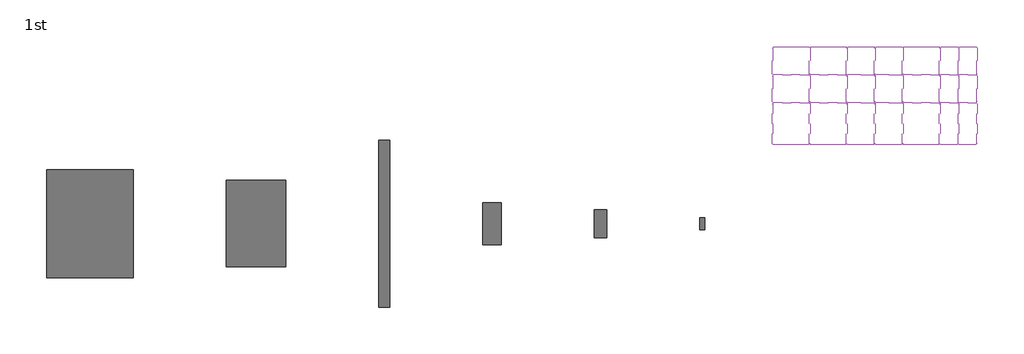
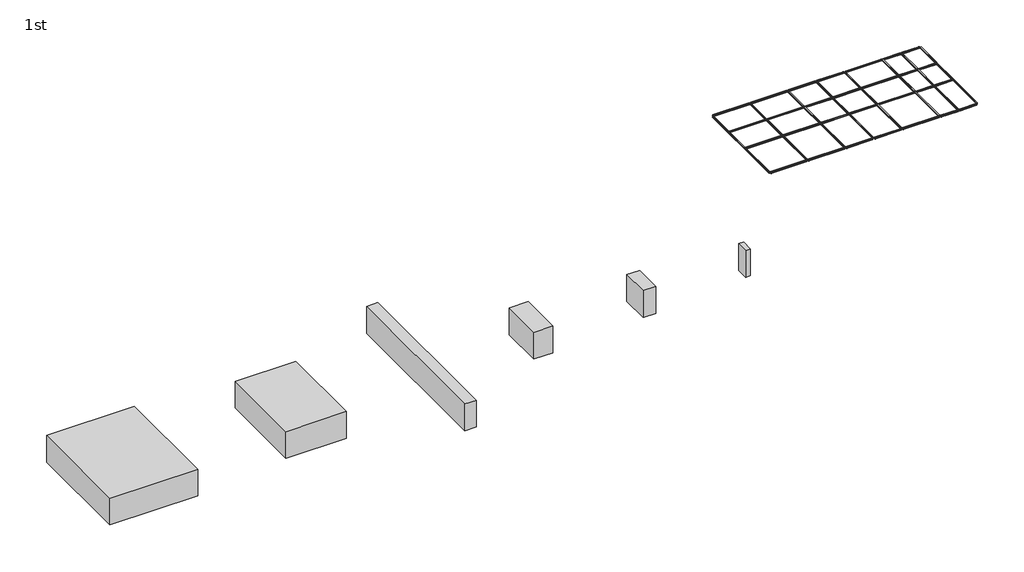
# One storey: 52 beams, 6 proxies.
"""IFC4 building model written with IfcOpenShell, lengths in millimetres."""

import ifcopenshell
import ifcopenshell.guid

model = None  # the IFC model being written
_history = None  # IfcOwnerHistory: only IFC2X3 demands one
_inside = {}  # id of a spatial element -> (the spatial element, [elements in it])
_under = {}  # id of a project, library or spatial element -> (it, [spatial elements below it])
_declared = {}  # id of a project -> (the project, [libraries it declares])
_typed = {}  # id of a type object -> (the type object, [elements of that type])
_made_of = {}  # id of a material, layer set ... -> (it, [elements and type objects made of it])


def new_model(schema):
    """Start an empty IFC model of exactly this schema.

    Asked for "IFC4X3", IfcOpenShell would pick the latest addendum, in which some entities
    have other attributes; the version numbers below select the first issue.
    IFC2X3 requires an IfcOwnerHistory on every rooted entity: one is made here for all.
    """
    global model, _history
    if schema == "IFC4X3":
        model = ifcopenshell.file(schema_version=(4, 3, 0, 0))
    else:
        model = ifcopenshell.file(schema=schema)
    _inside.clear()
    _under.clear()
    _declared.clear()
    _typed.clear()
    _made_of.clear()
    _history = None
    if model.schema == "IFC2X3":
        org = make("IfcOrganization", Name="unknown")
        user = make(
            "IfcPersonAndOrganization",
            ThePerson=make("IfcPerson", FamilyName="unknown"),
            TheOrganization=org,
        )
        app = make(
            "IfcApplication",
            ApplicationDeveloper=org,
            Version="unknown",
            ApplicationFullName="unknown",
            ApplicationIdentifier="unknown",
        )
        _history = make(
            "IfcOwnerHistory",
            OwningUser=user,
            OwningApplication=app,
            ChangeAction="ADDED",
            CreationDate=0,
        )
    return model


def make(cls, **values):
    """One entity of the class cls with the attributes given. An attribute that is None is left unset."""
    return model.create_entity(
        cls, **{name: value for name, value in values.items() if value is not None}
    )


def rooted(cls, **values):
    """An entity with a GlobalId (a new one), such as an element, a storey or a relation."""
    return make(cls, GlobalId=ifcopenshell.guid.new(), OwnerHistory=_history, **values)


def si_unit(unit_type, name, prefix=None):
    """IfcSIUnit, for example si_unit("LENGTHUNIT", "METRE", prefix="MILLI")."""
    return make("IfcSIUnit", UnitType=unit_type, Prefix=prefix, Name=name)


def assignment(units):
    """IfcUnitAssignment: the units of a project."""
    return None if units is None else make("IfcUnitAssignment", Units=units)


def point(xyz):
    """IfcCartesianPoint."""
    return None if xyz is None else make("IfcCartesianPoint", Coordinates=xyz)


def direction(xyz):
    """IfcDirection."""
    return None if xyz is None else make("IfcDirection", DirectionRatios=xyz)


def frame(location, z_axis=None, x_axis=None):
    """IfcAxis2Placement3D, a coordinate frame: its origin and axes. An axis left out is left unset."""
    return make(
        "IfcAxis2Placement3D",
        Location=point(location),
        Axis=direction(z_axis),
        RefDirection=direction(x_axis),
    )


def frame_2d(location, x_axis=None):
    """IfcAxis2Placement2D, a coordinate frame in the plane: its origin and x axis."""
    return make(
        "IfcAxis2Placement2D", Location=point(location), RefDirection=direction(x_axis)
    )


def origin():
    """The frame at (0, 0, 0) with its axes left unset."""
    return frame((0.0, 0.0, 0.0))


def origin_with_axes():
    """The frame at (0, 0, 0) with the z axis (0, 0, 1) and the x axis (1, 0, 0) written out."""
    return frame((0.0, 0.0, 0.0), z_axis=(0.0, 0.0, 1.0), x_axis=(1.0, 0.0, 0.0))


def place(relative_to, where):
    """IfcLocalPlacement: puts the frame where relative to a parent placement (None: the world)."""
    return make(
        "IfcLocalPlacement", PlacementRelTo=relative_to, RelativePlacement=where
    )


def context(
    kind, dimensions, precision=None, world=None, true_north=None, identifier=None
):
    """IfcGeometricRepresentationContext, for example the 3D "Model" context."""
    return make(
        "IfcGeometricRepresentationContext",
        ContextIdentifier=identifier,
        ContextType=kind,
        CoordinateSpaceDimension=dimensions,
        Precision=precision,
        WorldCoordinateSystem=world,
        TrueNorth=true_north,
    )


def project(units=None, contexts=None):
    """IfcProject with its units and contexts."""
    return rooted(
        "IfcProject",
        Name="project",
        RepresentationContexts=contexts,
        UnitsInContext=assignment(units),
    )


def spatial(cls, under=None, at=None, **own):
    """A site, building, storey or space (cls), placed at a placement, below another one or the project."""
    s = rooted(cls, ObjectPlacement=at, **own)
    if under is not None:
        _under.setdefault(under.id(), (under, []))[1].append(s)
    return s


def polyline(points):
    """IfcPolyline through the points."""
    return make("IfcPolyline", Points=[point(p) for p in points])


def circle_curve(where, radius):
    """IfcCircle in the frame where."""
    return make("IfcCircle", Position=where, Radius=radius)


def trimmed(basis, trim1, trim2, sense, master):
    """IfcTrimmedCurve: the piece of a basis curve between two trims."""
    return make(
        "IfcTrimmedCurve",
        BasisCurve=basis,
        Trim1=trim1,
        Trim2=trim2,
        SenseAgreement=sense,
        MasterRepresentation=master,
    )


def segment(curve, same_sense, transition):
    """IfcCompositeCurveSegment."""
    return make(
        "IfcCompositeCurveSegment",
        Transition=transition,
        SameSense=same_sense,
        ParentCurve=curve,
    )


def composite_curve(segments, self_intersect=None):
    """IfcCompositeCurve: segments joined end to end."""
    return make("IfcCompositeCurve", Segments=segments, SelfIntersect=self_intersect)


def outline(outer, holes=None, kind="AREA"):
    """IfcArbitraryClosedProfileDef: a profile drawn as a closed curve; with holes, ...WithVoids."""
    if holes is None:
        return make("IfcArbitraryClosedProfileDef", ProfileType=kind, OuterCurve=outer)
    return make(
        "IfcArbitraryProfileDefWithVoids",
        ProfileType=kind,
        OuterCurve=outer,
        InnerCurves=holes,
    )


def extrude(swept, where, along, depth):
    """IfcExtrudedAreaSolid: the profile swept, set in the frame where, extruded along a direction by depth."""
    return make(
        "IfcExtrudedAreaSolid",
        SweptArea=swept,
        Position=where,
        ExtrudedDirection=direction(along),
        Depth=depth,
    )


def shape(context_of_items, identifier, shape_type, items):
    """IfcShapeRepresentation: the items that make up one representation, for example the "Body"."""
    return make(
        "IfcShapeRepresentation",
        ContextOfItems=context_of_items,
        RepresentationIdentifier=identifier,
        RepresentationType=shape_type,
        Items=items,
    )


def source(mapping_origin, context_of_items, identifier, shape_type, items):
    """IfcRepresentationMap: a shape defined once, which mapped items show again and again."""
    return make(
        "IfcRepresentationMap",
        MappingOrigin=mapping_origin,
        MappedRepresentation=shape(context_of_items, identifier, shape_type, items),
    )


def transform(
    local_origin,
    x_axis=None,
    y_axis=None,
    z_axis=None,
    scale=None,
    scale2=None,
    scale3=None,
    uniform=True,
):
    """IfcCartesianTransformationOperator3D, or its non-uniform kind. x_axis, y_axis, z_axis: its Axis1, 2, 3."""
    if uniform:
        return make(
            "IfcCartesianTransformationOperator3D",
            Axis1=direction(x_axis),
            Axis2=direction(y_axis),
            LocalOrigin=point(local_origin),
            Scale=scale,
            Axis3=direction(z_axis),
        )
    return make(
        "IfcCartesianTransformationOperator3DnonUniform",
        Axis1=direction(x_axis),
        Axis2=direction(y_axis),
        LocalOrigin=point(local_origin),
        Scale=scale,
        Axis3=direction(z_axis),
        Scale2=scale2,
        Scale3=scale3,
    )


def mapped(mapping_source, mapping_target):
    """IfcMappedItem: shows the shape of a source again, moved by a transform."""
    return make(
        "IfcMappedItem", MappingSource=mapping_source, MappingTarget=mapping_target
    )


def made_of(thing, what):
    """Note that an element or type object is made of a material, layer set ...; save() writes the relation."""
    if what is not None:
        _made_of.setdefault(what.id(), (what, []))[1].append(thing)
    return thing


def element(
    cls,
    number,
    at=None,
    inside=None,
    cuts=None,
    type_object=None,
    material=None,
    context=None,
    identifier="Body",
    shape_type=None,
    held_by="IfcProductDefinitionShape",
    body=None,
    shapes=None,
    **own,
):
    """One element of the class cls, such as IfcWall. Its Tag is "e" and its number.

    at: its placement. inside: the storey or other place that contains it. cuts: it is an
    opening in that element (IfcRelVoidsElement). A single representation is given by context,
    identifier, shape_type and body (its items); several are given by shapes. held_by: the class
    of the entity that holds the representations. save() writes the other relations.
    """
    e = rooted(cls, Tag="e%d" % number, ObjectPlacement=at, **own)
    if body is not None:
        shapes = [shape(context, identifier, shape_type, body)]
    if shapes is not None:
        e.Representation = make(held_by, Representations=shapes)
    if inside is not None:
        _inside.setdefault(inside.id(), (inside, []))[1].append(e)
    if cuts is not None:
        rooted(
            "IfcRelVoidsElement", RelatingBuildingElement=cuts, RelatedOpeningElement=e
        )
    if type_object is not None:
        _typed.setdefault(type_object.id(), (type_object, []))[1].append(e)
    return made_of(e, material)


def aggregate(whole, parts):
    """IfcRelAggregates: a whole, such as a stair, and the parts it consists of."""
    return rooted("IfcRelAggregates", RelatingObject=whole, RelatedObjects=parts)


def save(model, path):
    """Write the relations noted so far, then the file.

    IfcRelAggregates (storeys below a building ...), IfcRelContainedInSpatialStructure (elements
    in a storey), IfcRelDefinesByType, IfcRelAssociatesMaterial and IfcRelDeclares: one each for
    every whole, place, type object, material and project.
    """
    for whole, parts in _under.values():
        aggregate(whole, parts)
    for where, things in _inside.values():
        rooted(
            "IfcRelContainedInSpatialStructure",
            RelatedElements=things,
            RelatingStructure=where,
        )
    for kind, things in _typed.values():
        rooted("IfcRelDefinesByType", RelatedObjects=things, RelatingType=kind)
    for what, things in _made_of.values():
        rooted("IfcRelAssociatesMaterial", RelatedObjects=things, RelatingMaterial=what)
    for by, libraries in _declared.values():
        rooted("IfcRelDeclares", RelatingContext=by, RelatedDefinitions=libraries)
    model.write(path)


def ub_universal_beams_ub305x165x40_6dcc7521(model_context):
    return source(origin(), model_context, "Body", "SweptSolid", [
        extrude(outline(composite_curve([segment(polyline([(82.5, -141.5), (82.5, -151.7), (-82.5, -151.7), (-82.5, -141.5), (-11.9, -141.5)]), True, "CONTINUOUS"), segment(trimmed(circle_curve(frame_2d((-11.9, -132.6)), 8.9), [point((-11.9, -141.5))], [point((-3.0, -132.6))], True, "CARTESIAN"), True, "CONTINUOUS"), segment(polyline([(-3.0, -132.6), (-3.0, 132.6)]), True, "CONTINUOUS"), segment(trimmed(circle_curve(frame_2d((-11.9, 132.6)), 8.9), [point((-3.0, 132.6))], [point((-11.9, 141.5))], True, "CARTESIAN"), True, "CONTINUOUS"), segment(polyline([(-11.9, 141.5), (-82.5, 141.5), (-82.5, 151.7), (82.5, 151.7), (82.5, 141.5), (11.9, 141.5)]), True, "CONTINUOUS"), segment(trimmed(circle_curve(frame_2d((11.9, 132.6)), 8.9), [point((11.9, 141.5))], [point((3.0, 132.6))], True, "CARTESIAN"), True, "CONTINUOUS"), segment(polyline([(3.0, 132.6), (3.0, -132.6)]), True, "CONTINUOUS"), segment(trimmed(circle_curve(frame_2d((11.9, -132.6)), 8.9), [point((3.0, -132.6))], [point((11.9, -141.5))], True, "CARTESIAN"), True, "CONTINUOUS"), segment(polyline([(11.9, -141.5), (82.5, -141.5)]), True, "CONTINUOUS")], self_intersect=False)), frame((-4333.3, 0.0, 0.0), z_axis=(1.0, 0.0, 0.0), x_axis=(0.0, 1.0, 0.0)), (0.0, 0.0, 1.0), 8666.6),
    ])


def ub_universal_beams_ub305x165x40_7f5f946b(model_context):
    return source(origin(), model_context, "Body", "SweptSolid", [
        extrude(outline(composite_curve([segment(polyline([(82.5, -141.5), (82.5, -151.7), (-82.5, -151.7), (-82.5, -141.5), (-11.9, -141.5)]), True, "CONTINUOUS"), segment(trimmed(circle_curve(frame_2d((-11.9, -132.6)), 8.9), [point((-11.9, -141.5))], [point((-3.0, -132.6))], True, "CARTESIAN"), True, "CONTINUOUS"), segment(polyline([(-3.0, -132.6), (-3.0, 132.6)]), True, "CONTINUOUS"), segment(trimmed(circle_curve(frame_2d((-11.9, 132.6)), 8.9), [point((-3.0, 132.6))], [point((-11.9, 141.5))], True, "CARTESIAN"), True, "CONTINUOUS"), segment(polyline([(-11.9, 141.5), (-82.5, 141.5), (-82.5, 151.7), (82.5, 151.7), (82.5, 141.5), (11.9, 141.5)]), True, "CONTINUOUS"), segment(trimmed(circle_curve(frame_2d((11.9, 132.6)), 8.9), [point((11.9, 141.5))], [point((3.0, 132.6))], True, "CARTESIAN"), True, "CONTINUOUS"), segment(polyline([(3.0, 132.6), (3.0, -132.6)]), True, "CONTINUOUS"), segment(trimmed(circle_curve(frame_2d((11.9, -132.6)), 8.9), [point((3.0, -132.6))], [point((11.9, -141.5))], True, "CARTESIAN"), True, "CONTINUOUS"), segment(polyline([(11.9, -141.5), (82.5, -141.5)]), True, "CONTINUOUS")], self_intersect=False)), frame((-2833.3, 0.0, 0.0), z_axis=(1.0, 0.0, 0.0), x_axis=(0.0, 1.0, 0.0)), (0.0, 0.0, 1.0), 5666.6),
    ])


def ub_universal_beams_ub305x165x40_37dc1813(model_context):
    return source(origin(), model_context, "Body", "SweptSolid", [
        extrude(outline(composite_curve([segment(polyline([(82.5, -141.5), (82.5, -151.7), (-82.5, -151.7), (-82.5, -141.5), (-11.9, -141.5)]), True, "CONTINUOUS"), segment(trimmed(circle_curve(frame_2d((-11.9, -132.6)), 8.9), [point((-11.9, -141.5))], [point((-3.0, -132.6))], True, "CARTESIAN"), True, "CONTINUOUS"), segment(polyline([(-3.0, -132.6), (-3.0, 132.6)]), True, "CONTINUOUS"), segment(trimmed(circle_curve(frame_2d((-11.9, 132.6)), 8.9), [point((-3.0, 132.6))], [point((-11.9, 141.5))], True, "CARTESIAN"), True, "CONTINUOUS"), segment(polyline([(-11.9, 141.5), (-82.5, 141.5), (-82.5, 151.7), (82.5, 151.7), (82.5, 141.5), (11.9, 141.5)]), True, "CONTINUOUS"), segment(trimmed(circle_curve(frame_2d((11.9, 132.6)), 8.9), [point((11.9, 141.5))], [point((3.0, 132.6))], True, "CARTESIAN"), True, "CONTINUOUS"), segment(polyline([(3.0, 132.6), (3.0, -132.6)]), True, "CONTINUOUS"), segment(trimmed(circle_curve(frame_2d((11.9, -132.6)), 8.9), [point((3.0, -132.6))], [point((11.9, -141.5))], True, "CARTESIAN"), True, "CONTINUOUS"), segment(polyline([(11.9, -141.5), (82.5, -141.5)]), True, "CONTINUOUS")], self_intersect=False)), frame((-3834.6, 0.0, 0.0), z_axis=(1.0, 0.0, 0.0), x_axis=(0.0, 1.0, 0.0)), (0.0, 0.0, 1.0), 7669.2),
    ])


def ub_universal_beams_ub305x165x40_4fbda082(model_context):
    return source(origin(), model_context, "Body", "SweptSolid", [
        extrude(outline(composite_curve([segment(polyline([(82.5, -141.5), (82.5, -151.7), (-82.5, -151.7), (-82.5, -141.5), (-11.9, -141.5)]), True, "CONTINUOUS"), segment(trimmed(circle_curve(frame_2d((-11.9, -132.6)), 8.9), [point((-11.9, -141.5))], [point((-3.0, -132.6))], True, "CARTESIAN"), True, "CONTINUOUS"), segment(polyline([(-3.0, -132.6), (-3.0, 132.6)]), True, "CONTINUOUS"), segment(trimmed(circle_curve(frame_2d((-11.9, 132.6)), 8.9), [point((-3.0, 132.6))], [point((-11.9, 141.5))], True, "CARTESIAN"), True, "CONTINUOUS"), segment(polyline([(-11.9, 141.5), (-82.5, 141.5), (-82.5, 151.7), (82.5, 151.7), (82.5, 141.5), (11.9, 141.5)]), True, "CONTINUOUS"), segment(trimmed(circle_curve(frame_2d((11.9, 132.6)), 8.9), [point((11.9, 141.5))], [point((3.0, 132.6))], True, "CARTESIAN"), True, "CONTINUOUS"), segment(polyline([(3.0, 132.6), (3.0, -132.6)]), True, "CONTINUOUS"), segment(trimmed(circle_curve(frame_2d((11.9, -132.6)), 8.9), [point((3.0, -132.6))], [point((11.9, -141.5))], True, "CARTESIAN"), True, "CONTINUOUS"), segment(polyline([(11.9, -141.5), (82.5, -141.5)]), True, "CONTINUOUS")], self_intersect=False)), frame((-2834.6, 0.0, 0.0), z_axis=(1.0, 0.0, 0.0), x_axis=(0.0, 1.0, 0.0)), (0.0, 0.0, 1.0), 5669.2),
    ])


def ub_universal_beams_ub305x165x40_037cda9e(model_context):
    return source(origin(), model_context, "Body", "SweptSolid", [
        extrude(outline(composite_curve([segment(polyline([(82.5, -141.5), (82.5, -151.7), (-82.5, -151.7), (-82.5, -141.5), (-11.9, -141.5)]), True, "CONTINUOUS"), segment(trimmed(circle_curve(frame_2d((-11.9, -132.6)), 8.9), [point((-11.9, -141.5))], [point((-3.0, -132.6))], True, "CARTESIAN"), True, "CONTINUOUS"), segment(polyline([(-3.0, -132.6), (-3.0, 132.6)]), True, "CONTINUOUS"), segment(trimmed(circle_curve(frame_2d((-11.9, 132.6)), 8.9), [point((-3.0, 132.6))], [point((-11.9, 141.5))], True, "CARTESIAN"), True, "CONTINUOUS"), segment(polyline([(-11.9, 141.5), (-82.5, 141.5), (-82.5, 151.7), (82.5, 151.7), (82.5, 141.5), (11.9, 141.5)]), True, "CONTINUOUS"), segment(trimmed(circle_curve(frame_2d((11.9, 132.6)), 8.9), [point((11.9, 141.5))], [point((3.0, 132.6))], True, "CARTESIAN"), True, "CONTINUOUS"), segment(polyline([(3.0, 132.6), (3.0, -132.6)]), True, "CONTINUOUS"), segment(trimmed(circle_curve(frame_2d((11.9, -132.6)), 8.9), [point((3.0, -132.6))], [point((11.9, -141.5))], True, "CARTESIAN"), True, "CONTINUOUS"), segment(polyline([(11.9, -141.5), (82.5, -141.5)]), True, "CONTINUOUS")], self_intersect=False)), frame((-1834.6, 0.0, 0.0), z_axis=(1.0, 0.0, 0.0), x_axis=(0.0, 1.0, 0.0)), (0.0, 0.0, 1.0), 3669.2),
    ])


def generic_models_29bcd6f9(model_context):
    return source(origin(), model_context, "Body", "SweptSolid", [
        extrude(outline(polyline([(2000.0, 4500.0), (2000.0, -4500.0), (-2000.0, -4500.0), (-2000.0, 4500.0), (2000.0, 4500.0)])), origin_with_axes(), (0.0, 0.0, 1.0), 6000.0),
    ])


def generic_models_d82b1902(model_context):
    return source(origin(), model_context, "Body", "SweptSolid", [
        extrude(outline(polyline([(9300.0, 11600.0), (9300.0, -11600.0), (-9300.0, -11600.0), (-9300.0, 11600.0), (9300.0, 11600.0)])), origin_with_axes(), (0.0, 0.0, 1.0), 6000.0),
    ])


def generic_models_21711933(model_context):
    return source(origin(), model_context, "Body", "SweptSolid", [
        extrude(outline(polyline([(6400.0, 9300.0), (6400.0, -9300.0), (-6400.0, -9300.0), (-6400.0, 9300.0), (6400.0, 9300.0)])), origin_with_axes(), (0.0, 0.0, 1.0), 6000.0),
    ])


def generic_models_03d31222(model_context):
    return source(origin(), model_context, "Body", "SweptSolid", [
        extrude(outline(polyline([(1200.0, 18000.0), (1200.0, -18000.0), (-1200.0, -18000.0), (-1200.0, 18000.0), (1200.0, 18000.0)])), origin_with_axes(), (0.0, 0.0, 1.0), 6000.0),
    ])


def generic_models_5634f436(model_context):
    return source(origin(), model_context, "Body", "SweptSolid", [
        extrude(outline(polyline([(1350.0, 3000.0), (1350.0, -3000.0), (-1350.0, -3000.0), (-1350.0, 3000.0), (1350.0, 3000.0)])), origin_with_axes(), (0.0, 0.0, 1.0), 6000.0),
    ])


def generic_models_71e2440f(model_context):
    return source(origin(), model_context, "Body", "SweptSolid", [
        extrude(outline(polyline([(500.0, 1250.0), (500.0, -1250.0), (-500.0, -1250.0), (-500.0, 1250.0), (500.0, 1250.0)])), origin_with_axes(), (0.0, 0.0, 1.0), 6000.0),
    ])


model = new_model("IFC4")

# Units and contexts
model_context = context("Model", 3, world=origin())
ifc_project = project(units=[si_unit("LENGTHUNIT", "METRE", prefix="MILLI")], contexts=[model_context])

# Site, building, storey
site = spatial("IfcSite", under=ifc_project)
building = spatial("IfcBuilding", under=site)
storey = spatial("IfcBuildingStorey", under=building, Name="1st", Elevation=7000.0)

# Beams
placement = place(None, origin())
ub_universal_beams_ub305x165x40_shape = ub_universal_beams_ub305x165x40_6dcc7521(model_context)
element("IfcBeam", 1, ObjectType="UB-Universal Beams : UB305x165x40", at=placement, inside=storey, context=model_context, shape_type="MappedRepresentation", body=[
    mapped(ub_universal_beams_ub305x165x40_shape, transform((156114.1020501, 135515.7581198, 13848.3), x_axis=(0.0, 1.0, 0.0), y_axis=(-1.0, 0.0, 0.0), z_axis=(0.0, 0.0, 1.0))),
])
element("IfcBeam", 2, ObjectType="UB-Universal Beams : UB305x165x40", at=placement, inside=storey, context=model_context, shape_type="MappedRepresentation", body=[
    mapped(ub_universal_beams_ub305x165x40_shape, transform((164114.1020501, 135515.7581198, 13848.3), x_axis=(0.0, 1.0, 0.0), y_axis=(-1.0, 0.0, 0.0), z_axis=(0.0, 0.0, 1.0))),
])
element("IfcBeam", 3, ObjectType="UB-Universal Beams : UB305x165x40", at=placement, inside=storey, context=model_context, shape_type="MappedRepresentation", body=[
    mapped(ub_universal_beams_ub305x165x40_shape, transform((172114.1020501, 135515.7581198, 13848.3), x_axis=(0.0, 1.0, 0.0), y_axis=(-1.0, 0.0, 0.0), z_axis=(0.0, 0.0, 1.0))),
])
element("IfcBeam", 4, ObjectType="UB-Universal Beams : UB305x165x40", at=placement, inside=storey, context=model_context, shape_type="MappedRepresentation", body=[
    mapped(ub_universal_beams_ub305x165x40_shape, transform((178114.1020501, 135515.7581198, 13848.3), x_axis=(0.0, 1.0, 0.0), y_axis=(-1.0, 0.0, 0.0), z_axis=(0.0, 0.0, 1.0))),
])
element("IfcBeam", 5, ObjectType="UB-Universal Beams : UB305x165x40", at=placement, inside=storey, context=model_context, shape_type="MappedRepresentation", body=[
    mapped(ub_universal_beams_ub305x165x40_shape, transform((184114.1020501, 135515.7581198, 13848.3), x_axis=(0.0, 1.0, 0.0), y_axis=(-1.0, 0.0, 0.0), z_axis=(0.0, 0.0, 1.0))),
])
element("IfcBeam", 6, ObjectType="UB-Universal Beams : UB305x165x40", at=placement, inside=storey, context=model_context, shape_type="MappedRepresentation", body=[
    mapped(ub_universal_beams_ub305x165x40_shape, transform((192114.1020501, 135515.7581198, 13848.3), x_axis=(0.0, 1.0, 0.0), y_axis=(-1.0, 0.0, 0.0), z_axis=(0.0, 0.0, 1.0))),
])
element("IfcBeam", 7, ObjectType="UB-Universal Beams : UB305x165x40", at=placement, inside=storey, context=model_context, shape_type="MappedRepresentation", body=[
    mapped(ub_universal_beams_ub305x165x40_shape, transform((196114.1020501, 135515.7581198, 13848.3), x_axis=(0.0, 1.0, 0.0), y_axis=(-1.0, 0.0, 0.0), z_axis=(0.0, 0.0, 1.0))),
])
element("IfcBeam", 8, ObjectType="UB-Universal Beams : UB305x165x40", at=placement, inside=storey, context=model_context, shape_type="MappedRepresentation", body=[
    mapped(ub_universal_beams_ub305x165x40_shape, transform((200114.1020501, 135515.7581198, 13848.3), x_axis=(0.0, 1.0, 0.0), y_axis=(-1.0, 0.0, 0.0), z_axis=(0.0, 0.0, 1.0))),
])
ub_universal_beams_ub305x165x40_2_shape = ub_universal_beams_ub305x165x40_7f5f946b(model_context)
element("IfcBeam", 9, ObjectType="UB-Universal Beams : UB305x165x40", at=placement, inside=storey, context=model_context, shape_type="MappedRepresentation", body=[
    mapped(ub_universal_beams_ub305x165x40_2_shape, transform((156114.1020501, 143015.7581198, 13848.3), x_axis=(0.0, 1.0, 0.0), y_axis=(-1.0, 0.0, 0.0), z_axis=(0.0, 0.0, 1.0))),
])
element("IfcBeam", 10, ObjectType="UB-Universal Beams : UB305x165x40", at=placement, inside=storey, context=model_context, shape_type="MappedRepresentation", body=[
    mapped(ub_universal_beams_ub305x165x40_2_shape, transform((156114.1020501, 149015.7581198, 13848.3), x_axis=(0.0, 1.0, 0.0), y_axis=(-1.0, 0.0, 0.0), z_axis=(0.0, 0.0, 1.0))),
])
element("IfcBeam", 11, ObjectType="UB-Universal Beams : UB305x165x40", at=placement, inside=storey, context=model_context, shape_type="MappedRepresentation", body=[
    mapped(ub_universal_beams_ub305x165x40_2_shape, transform((164114.1020501, 143015.7581198, 13848.3), x_axis=(0.0, 1.0, 0.0), y_axis=(-1.0, 0.0, 0.0), z_axis=(0.0, 0.0, 1.0))),
])
element("IfcBeam", 12, ObjectType="UB-Universal Beams : UB305x165x40", at=placement, inside=storey, context=model_context, shape_type="MappedRepresentation", body=[
    mapped(ub_universal_beams_ub305x165x40_2_shape, transform((164114.1020501, 149015.7581198, 13848.3), x_axis=(0.0, 1.0, 0.0), y_axis=(-1.0, 0.0, 0.0), z_axis=(0.0, 0.0, 1.0))),
])
element("IfcBeam", 13, ObjectType="UB-Universal Beams : UB305x165x40", at=placement, inside=storey, context=model_context, shape_type="MappedRepresentation", body=[
    mapped(ub_universal_beams_ub305x165x40_2_shape, transform((172114.1020501, 143015.7581198, 13848.3), x_axis=(0.0, 1.0, 0.0), y_axis=(-1.0, 0.0, 0.0), z_axis=(0.0, 0.0, 1.0))),
])
element("IfcBeam", 14, ObjectType="UB-Universal Beams : UB305x165x40", at=placement, inside=storey, context=model_context, shape_type="MappedRepresentation", body=[
    mapped(ub_universal_beams_ub305x165x40_2_shape, transform((172114.1020501, 149015.7581198, 13848.3), x_axis=(0.0, 1.0, 0.0), y_axis=(-1.0, 0.0, 0.0), z_axis=(0.0, 0.0, 1.0))),
])
element("IfcBeam", 15, ObjectType="UB-Universal Beams : UB305x165x40", at=placement, inside=storey, context=model_context, shape_type="MappedRepresentation", body=[
    mapped(ub_universal_beams_ub305x165x40_2_shape, transform((178114.1020501, 143015.7581198, 13848.3), x_axis=(0.0, 1.0, 0.0), y_axis=(-1.0, 0.0, 0.0), z_axis=(0.0, 0.0, 1.0))),
])
element("IfcBeam", 16, ObjectType="UB-Universal Beams : UB305x165x40", at=placement, inside=storey, context=model_context, shape_type="MappedRepresentation", body=[
    mapped(ub_universal_beams_ub305x165x40_2_shape, transform((178114.1020501, 149015.7581198, 13848.3), x_axis=(0.0, 1.0, 0.0), y_axis=(-1.0, 0.0, 0.0), z_axis=(0.0, 0.0, 1.0))),
])
element("IfcBeam", 17, ObjectType="UB-Universal Beams : UB305x165x40", at=placement, inside=storey, context=model_context, shape_type="MappedRepresentation", body=[
    mapped(ub_universal_beams_ub305x165x40_2_shape, transform((184114.1020501, 143015.7581198, 13848.3), x_axis=(0.0, 1.0, 0.0), y_axis=(-1.0, 0.0, 0.0), z_axis=(0.0, 0.0, 1.0))),
])
element("IfcBeam", 18, ObjectType="UB-Universal Beams : UB305x165x40", at=placement, inside=storey, context=model_context, shape_type="MappedRepresentation", body=[
    mapped(ub_universal_beams_ub305x165x40_2_shape, transform((184114.1020501, 149015.7581198, 13848.3), x_axis=(0.0, 1.0, 0.0), y_axis=(-1.0, 0.0, 0.0), z_axis=(0.0, 0.0, 1.0))),
])
element("IfcBeam", 19, ObjectType="UB-Universal Beams : UB305x165x40", at=placement, inside=storey, context=model_context, shape_type="MappedRepresentation", body=[
    mapped(ub_universal_beams_ub305x165x40_2_shape, transform((192114.1020501, 143015.7581198, 13848.3), x_axis=(0.0, 1.0, 0.0), y_axis=(-1.0, 0.0, 0.0), z_axis=(0.0, 0.0, 1.0))),
])
element("IfcBeam", 20, ObjectType="UB-Universal Beams : UB305x165x40", at=placement, inside=storey, context=model_context, shape_type="MappedRepresentation", body=[
    mapped(ub_universal_beams_ub305x165x40_2_shape, transform((192114.1020501, 149015.7581198, 13848.3), x_axis=(0.0, 1.0, 0.0), y_axis=(-1.0, 0.0, 0.0), z_axis=(0.0, 0.0, 1.0))),
])
element("IfcBeam", 21, ObjectType="UB-Universal Beams : UB305x165x40", at=placement, inside=storey, context=model_context, shape_type="MappedRepresentation", body=[
    mapped(ub_universal_beams_ub305x165x40_2_shape, transform((196114.1020501, 143015.7581198, 13848.3), x_axis=(0.0, 1.0, 0.0), y_axis=(-1.0, 0.0, 0.0), z_axis=(0.0, 0.0, 1.0))),
])
element("IfcBeam", 22, ObjectType="UB-Universal Beams : UB305x165x40", at=placement, inside=storey, context=model_context, shape_type="MappedRepresentation", body=[
    mapped(ub_universal_beams_ub305x165x40_2_shape, transform((196114.1020501, 149015.7581198, 13848.3), x_axis=(0.0, 1.0, 0.0), y_axis=(-1.0, 0.0, 0.0), z_axis=(0.0, 0.0, 1.0))),
])
element("IfcBeam", 23, ObjectType="UB-Universal Beams : UB305x165x40", at=placement, inside=storey, context=model_context, shape_type="MappedRepresentation", body=[
    mapped(ub_universal_beams_ub305x165x40_2_shape, transform((200114.1020501, 143015.7581198, 13848.3), x_axis=(0.0, 1.0, 0.0), y_axis=(-1.0, 0.0, 0.0), z_axis=(0.0, 0.0, 1.0))),
])
element("IfcBeam", 24, ObjectType="UB-Universal Beams : UB305x165x40", at=placement, inside=storey, context=model_context, shape_type="MappedRepresentation", body=[
    mapped(ub_universal_beams_ub305x165x40_2_shape, transform((200114.1020501, 149015.7581198, 13848.3), x_axis=(0.0, 1.0, 0.0), y_axis=(-1.0, 0.0, 0.0), z_axis=(0.0, 0.0, 1.0))),
])
ub_universal_beams_ub305x165x40_3_shape = ub_universal_beams_ub305x165x40_37dc1813(model_context)
element("IfcBeam", 25, ObjectType="UB-Universal Beams : UB305x165x40", at=placement, inside=storey, context=model_context, shape_type="MappedRepresentation", body=[
    mapped(ub_universal_beams_ub305x165x40_3_shape, transform((160114.1020501, 152015.7581198, 13848.3), x_axis=(1.0, 0.0, 0.0), y_axis=(0.0, 1.0, 0.0), z_axis=(0.0, 0.0, 1.0))),
])
element("IfcBeam", 26, ObjectType="UB-Universal Beams : UB305x165x40", at=placement, inside=storey, context=model_context, shape_type="MappedRepresentation", body=[
    mapped(ub_universal_beams_ub305x165x40_3_shape, transform((168114.1020501, 152015.7581198, 13848.3), x_axis=(1.0, 0.0, 0.0), y_axis=(0.0, 1.0, 0.0), z_axis=(0.0, 0.0, 1.0))),
])
element("IfcBeam", 27, ObjectType="UB-Universal Beams : UB305x165x40", at=placement, inside=storey, context=model_context, shape_type="MappedRepresentation", body=[
    mapped(ub_universal_beams_ub305x165x40_3_shape, transform((188114.1020501, 152015.7581198, 13848.3), x_axis=(1.0, 0.0, 0.0), y_axis=(0.0, 1.0, 0.0), z_axis=(0.0, 0.0, 1.0))),
])
element("IfcBeam", 28, ObjectType="UB-Universal Beams : UB305x165x40", at=placement, inside=storey, context=model_context, shape_type="MappedRepresentation", body=[
    mapped(ub_universal_beams_ub305x165x40_3_shape, transform((160114.1020501, 146015.7581198, 13848.3), x_axis=(1.0, 0.0, 0.0), y_axis=(0.0, 1.0, 0.0), z_axis=(0.0, 0.0, 1.0))),
])
element("IfcBeam", 29, ObjectType="UB-Universal Beams : UB305x165x40", at=placement, inside=storey, context=model_context, shape_type="MappedRepresentation", body=[
    mapped(ub_universal_beams_ub305x165x40_3_shape, transform((168114.1020501, 146015.7581198, 13848.3), x_axis=(1.0, 0.0, 0.0), y_axis=(0.0, 1.0, 0.0), z_axis=(0.0, 0.0, 1.0))),
])
element("IfcBeam", 30, ObjectType="UB-Universal Beams : UB305x165x40", at=placement, inside=storey, context=model_context, shape_type="MappedRepresentation", body=[
    mapped(ub_universal_beams_ub305x165x40_3_shape, transform((188114.1020501, 146015.7581198, 13848.3), x_axis=(1.0, 0.0, 0.0), y_axis=(0.0, 1.0, 0.0), z_axis=(0.0, 0.0, 1.0))),
])
element("IfcBeam", 31, ObjectType="UB-Universal Beams : UB305x165x40", at=placement, inside=storey, context=model_context, shape_type="MappedRepresentation", body=[
    mapped(ub_universal_beams_ub305x165x40_3_shape, transform((160114.1020501, 140015.7581198, 13848.3), x_axis=(1.0, 0.0, 0.0), y_axis=(0.0, 1.0, 0.0), z_axis=(0.0, 0.0, 1.0))),
])
element("IfcBeam", 32, ObjectType="UB-Universal Beams : UB305x165x40", at=placement, inside=storey, context=model_context, shape_type="MappedRepresentation", body=[
    mapped(ub_universal_beams_ub305x165x40_3_shape, transform((168114.1020501, 140015.7581198, 13848.3), x_axis=(1.0, 0.0, 0.0), y_axis=(0.0, 1.0, 0.0), z_axis=(0.0, 0.0, 1.0))),
])
element("IfcBeam", 33, ObjectType="UB-Universal Beams : UB305x165x40", at=placement, inside=storey, context=model_context, shape_type="MappedRepresentation", body=[
    mapped(ub_universal_beams_ub305x165x40_3_shape, transform((188114.1020501, 140015.7581198, 13848.3), x_axis=(1.0, 0.0, 0.0), y_axis=(0.0, 1.0, 0.0), z_axis=(0.0, 0.0, 1.0))),
])
element("IfcBeam", 34, ObjectType="UB-Universal Beams : UB305x165x40", at=placement, inside=storey, context=model_context, shape_type="MappedRepresentation", body=[
    mapped(ub_universal_beams_ub305x165x40_3_shape, transform((160114.1020501, 131015.7581198, 13848.3), x_axis=(1.0, 0.0, 0.0), y_axis=(0.0, 1.0, 0.0), z_axis=(0.0, 0.0, 1.0))),
])
element("IfcBeam", 35, ObjectType="UB-Universal Beams : UB305x165x40", at=placement, inside=storey, context=model_context, shape_type="MappedRepresentation", body=[
    mapped(ub_universal_beams_ub305x165x40_3_shape, transform((168114.1020501, 131015.7581198, 13848.3), x_axis=(1.0, 0.0, 0.0), y_axis=(0.0, 1.0, 0.0), z_axis=(0.0, 0.0, 1.0))),
])
element("IfcBeam", 36, ObjectType="UB-Universal Beams : UB305x165x40", at=placement, inside=storey, context=model_context, shape_type="MappedRepresentation", body=[
    mapped(ub_universal_beams_ub305x165x40_3_shape, transform((188114.1020501, 131015.7581198, 13848.3), x_axis=(1.0, 0.0, 0.0), y_axis=(0.0, 1.0, 0.0), z_axis=(0.0, 0.0, 1.0))),
])
ub_universal_beams_ub305x165x40_4_shape = ub_universal_beams_ub305x165x40_4fbda082(model_context)
element("IfcBeam", 37, ObjectType="UB-Universal Beams : UB305x165x40", at=placement, inside=storey, context=model_context, shape_type="MappedRepresentation", body=[
    mapped(ub_universal_beams_ub305x165x40_4_shape, transform((175114.1020501, 152015.7581198, 13848.3), x_axis=(1.0, 0.0, 0.0), y_axis=(0.0, 1.0, 0.0), z_axis=(0.0, 0.0, 1.0))),
])
element("IfcBeam", 38, ObjectType="UB-Universal Beams : UB305x165x40", at=placement, inside=storey, context=model_context, shape_type="MappedRepresentation", body=[
    mapped(ub_universal_beams_ub305x165x40_4_shape, transform((181114.1020501, 152015.7581198, 13848.3), x_axis=(1.0, 0.0, 0.0), y_axis=(0.0, 1.0, 0.0), z_axis=(0.0, 0.0, 1.0))),
])
element("IfcBeam", 39, ObjectType="UB-Universal Beams : UB305x165x40", at=placement, inside=storey, context=model_context, shape_type="MappedRepresentation", body=[
    mapped(ub_universal_beams_ub305x165x40_4_shape, transform((175114.1020501, 146015.7581198, 13848.3), x_axis=(1.0, 0.0, 0.0), y_axis=(0.0, 1.0, 0.0), z_axis=(0.0, 0.0, 1.0))),
])
element("IfcBeam", 40, ObjectType="UB-Universal Beams : UB305x165x40", at=placement, inside=storey, context=model_context, shape_type="MappedRepresentation", body=[
    mapped(ub_universal_beams_ub305x165x40_4_shape, transform((181114.1020501, 146015.7581198, 13848.3), x_axis=(1.0, 0.0, 0.0), y_axis=(0.0, 1.0, 0.0), z_axis=(0.0, 0.0, 1.0))),
])
element("IfcBeam", 41, ObjectType="UB-Universal Beams : UB305x165x40", at=placement, inside=storey, context=model_context, shape_type="MappedRepresentation", body=[
    mapped(ub_universal_beams_ub305x165x40_4_shape, transform((175114.1020501, 140015.7581198, 13848.3), x_axis=(1.0, 0.0, 0.0), y_axis=(0.0, 1.0, 0.0), z_axis=(0.0, 0.0, 1.0))),
])
element("IfcBeam", 42, ObjectType="UB-Universal Beams : UB305x165x40", at=placement, inside=storey, context=model_context, shape_type="MappedRepresentation", body=[
    mapped(ub_universal_beams_ub305x165x40_4_shape, transform((181114.1020501, 140015.7581198, 13848.3), x_axis=(1.0, 0.0, 0.0), y_axis=(0.0, 1.0, 0.0), z_axis=(0.0, 0.0, 1.0))),
])
element("IfcBeam", 43, ObjectType="UB-Universal Beams : UB305x165x40", at=placement, inside=storey, context=model_context, shape_type="MappedRepresentation", body=[
    mapped(ub_universal_beams_ub305x165x40_4_shape, transform((175114.1020501, 131015.7581198, 13848.3), x_axis=(1.0, 0.0, 0.0), y_axis=(0.0, 1.0, 0.0), z_axis=(0.0, 0.0, 1.0))),
])
element("IfcBeam", 44, ObjectType="UB-Universal Beams : UB305x165x40", at=placement, inside=storey, context=model_context, shape_type="MappedRepresentation", body=[
    mapped(ub_universal_beams_ub305x165x40_4_shape, transform((181114.1020501, 131015.7581198, 13848.3), x_axis=(1.0, 0.0, 0.0), y_axis=(0.0, 1.0, 0.0), z_axis=(0.0, 0.0, 1.0))),
])
ub_universal_beams_ub305x165x40_5_shape = ub_universal_beams_ub305x165x40_037cda9e(model_context)
element("IfcBeam", 45, ObjectType="UB-Universal Beams : UB305x165x40", at=placement, inside=storey, context=model_context, shape_type="MappedRepresentation", body=[
    mapped(ub_universal_beams_ub305x165x40_5_shape, transform((194114.1020501, 152015.7581198, 13848.3), x_axis=(1.0, 0.0, 0.0), y_axis=(0.0, 1.0, 0.0), z_axis=(0.0, 0.0, 1.0))),
])
element("IfcBeam", 46, ObjectType="UB-Universal Beams : UB305x165x40", at=placement, inside=storey, context=model_context, shape_type="MappedRepresentation", body=[
    mapped(ub_universal_beams_ub305x165x40_5_shape, transform((198114.1020501, 152015.7581198, 13848.3), x_axis=(1.0, 0.0, 0.0), y_axis=(0.0, 1.0, 0.0), z_axis=(0.0, 0.0, 1.0))),
])
element("IfcBeam", 47, ObjectType="UB-Universal Beams : UB305x165x40", at=placement, inside=storey, context=model_context, shape_type="MappedRepresentation", body=[
    mapped(ub_universal_beams_ub305x165x40_5_shape, transform((194114.1020501, 146015.7581198, 13848.3), x_axis=(1.0, 0.0, 0.0), y_axis=(0.0, 1.0, 0.0), z_axis=(0.0, 0.0, 1.0))),
])
element("IfcBeam", 48, ObjectType="UB-Universal Beams : UB305x165x40", at=placement, inside=storey, context=model_context, shape_type="MappedRepresentation", body=[
    mapped(ub_universal_beams_ub305x165x40_5_shape, transform((198114.1020501, 146015.7581198, 13848.3), x_axis=(1.0, 0.0, 0.0), y_axis=(0.0, 1.0, 0.0), z_axis=(0.0, 0.0, 1.0))),
])
element("IfcBeam", 49, ObjectType="UB-Universal Beams : UB305x165x40", at=placement, inside=storey, context=model_context, shape_type="MappedRepresentation", body=[
    mapped(ub_universal_beams_ub305x165x40_5_shape, transform((194114.1020501, 140015.7581198, 13848.3), x_axis=(1.0, 0.0, 0.0), y_axis=(0.0, 1.0, 0.0), z_axis=(0.0, 0.0, 1.0))),
])
element("IfcBeam", 50, ObjectType="UB-Universal Beams : UB305x165x40", at=placement, inside=storey, context=model_context, shape_type="MappedRepresentation", body=[
    mapped(ub_universal_beams_ub305x165x40_5_shape, transform((198114.1020501, 140015.7581198, 13848.3), x_axis=(1.0, 0.0, 0.0), y_axis=(0.0, 1.0, 0.0), z_axis=(0.0, 0.0, 1.0))),
])
element("IfcBeam", 51, ObjectType="UB-Universal Beams : UB305x165x40", at=placement, inside=storey, context=model_context, shape_type="MappedRepresentation", body=[
    mapped(ub_universal_beams_ub305x165x40_5_shape, transform((194114.1020501, 131015.7581198, 13848.3), x_axis=(1.0, 0.0, 0.0), y_axis=(0.0, 1.0, 0.0), z_axis=(0.0, 0.0, 1.0))),
])
element("IfcBeam", 52, ObjectType="UB-Universal Beams : UB305x165x40", at=placement, inside=storey, context=model_context, shape_type="MappedRepresentation", body=[
    mapped(ub_universal_beams_ub305x165x40_5_shape, transform((198114.1020501, 131015.7581198, 13848.3), x_axis=(1.0, 0.0, 0.0), y_axis=(0.0, 1.0, 0.0), z_axis=(0.0, 0.0, 1.0))),
])

# Proxies
generic_models_shape = generic_models_29bcd6f9(model_context)
element("IfcBuildingElementProxy", 53, Name="Space Planning Box_hec : Space Planning Box_hec", ObjectType="Space Planning Box_hec : Space Planning Box_hec", at=placement, inside=storey, context=model_context, shape_type="MappedRepresentation", body=[
    mapped(generic_models_shape, transform((95800.0, 114000.0, 7000.0), x_axis=(1.0, 0.0, 0.0), y_axis=(0.0, 1.0, 0.0), z_axis=(0.0, 0.0, 1.0))),
])
generic_models_2_shape = generic_models_d82b1902(model_context)
element("IfcBuildingElementProxy", 54, Name="Space Planning Box_hec : Space Planning Box_hec", ObjectType="Space Planning Box_hec : Space Planning Box_hec", at=placement, inside=storey, context=model_context, shape_type="MappedRepresentation", body=[
    mapped(generic_models_2_shape, transform((9300.0, 114000.0, 7000.0), x_axis=(1.0, 0.0, 0.0), y_axis=(0.0, 1.0, 0.0), z_axis=(0.0, 0.0, 1.0))),
])
generic_models_3_shape = generic_models_21711933(model_context)
element("IfcBuildingElementProxy", 55, Name="Space Planning Box_hec : Space Planning Box_hec", ObjectType="Space Planning Box_hec : Space Planning Box_hec", at=placement, inside=storey, context=model_context, shape_type="MappedRepresentation", body=[
    mapped(generic_models_3_shape, transform((45000.0, 114000.0, 7000.0), x_axis=(1.0, 0.0, 0.0), y_axis=(0.0, 1.0, 0.0), z_axis=(0.0, 0.0, 1.0))),
])
generic_models_4_shape = generic_models_03d31222(model_context)
element("IfcBuildingElementProxy", 56, Name="Space Planning Box_hec : Space Planning Box_hec", ObjectType="Space Planning Box_hec : Space Planning Box_hec", at=placement, inside=storey, context=model_context, shape_type="MappedRepresentation", body=[
    mapped(generic_models_4_shape, transform((72600.0, 114000.0, 7000.0), x_axis=(1.0, 0.0, 0.0), y_axis=(0.0, 1.0, 0.0), z_axis=(0.0, 0.0, 1.0))),
])
generic_models_5_shape = generic_models_5634f436(model_context)
element("IfcBuildingElementProxy", 57, Name="Space Planning Box_hec : Space Planning Box_hec", ObjectType="Space Planning Box_hec : Space Planning Box_hec", at=placement, inside=storey, context=model_context, shape_type="MappedRepresentation", body=[
    mapped(generic_models_5_shape, transform((119150.0, 114000.0, 7000.0), x_axis=(1.0, 0.0, 0.0), y_axis=(0.0, 1.0, 0.0), z_axis=(0.0, 0.0, 1.0))),
])
generic_models_6_shape = generic_models_71e2440f(model_context)
element("IfcBuildingElementProxy", 58, Name="Space Planning Box_hec : Space Planning Box_hec", ObjectType="Space Planning Box_hec : Space Planning Box_hec", at=placement, inside=storey, context=model_context, shape_type="MappedRepresentation", body=[
    mapped(generic_models_6_shape, transform((141000.0, 114000.0, 7000.0), x_axis=(1.0, 0.0, 0.0), y_axis=(0.0, 1.0, 0.0), z_axis=(0.0, 0.0, 1.0))),
])

save(model, "model.ifc")

# Revit data of these elements
# Type "UB-Universal Beams : UB305x165x40"
#   Section Name Key = "UB305X165X40"
#   Width = 16.5 cm
#   Web Thickness = 0.6 cm
#   Web Fillet = 0.89 cm
#   Warping Constant = 164000.0 cm⁶
#   Torsional Moment of Inertia = 14.70 cm⁴
#   Section Area = 51.3 cm²
#   Plastic Modulus weak axis = 142.0 cm³
#   Plastic Modulus strong axis = 623.0 cm³
#   Nominal Weight = 40.2999 kgf/m
#   Moment of Inertia weak axis = 764.00 cm⁴
#   Moment of Inertia strong axis = 8503.00 cm⁴
#   Height = 30.34 cm
#   Flange Thickness = 1.02 cm
#   Elastic Modulus weak axis = 92.6 cm³
#   Elastic Modulus strong axis = 560.0 cm³
#   Centroid Vertical = 15.17 cm
#   Centroid Horizontal = 8.25 cm
#   Bolt Spacing = 9.0 cm
#   Length [instance default] = 1500 mm
#   Structural Material [instance default] = Metal - Steel 43-275
#   Type Comments = ""
#   Assembly Code = ""
# Type "Space Planning Box_hec : Space Planning Box_hec"
#   Type Comments = "..."
#   Room Name [instance default] = "?"
#   Interior Finish [instance default] = ""
#   Exterior Finish [instance default] = ""
#   Department [instance default] = ""
#   Assembly Code = "..."
#   Width [instance default] = 1524 mm
#   Program Area [instance default] = 0 m²
#   Length [instance default] = 1524 mm
#   Height [instance default] = 1524 mm
#   Area [instance default] = 2.32258 m²
#   Fill Color [instance default] = Cyan
#   Default Elevation = 0
# Elements 1, 2, 3, 4, 5, 6, 7, 8, 9, 10, 11, 12, 13, 14, 15, 16, 17, 18, 19, 20, 21, 22, 23, 24, 25, 26, 27, 28, 29, 30, 31, 32, 33, 34, 35, 36, 37, 38, 39, 40, 41, 42, 43, 44, 45, 46, 47, 48, 49, 50, 51, 52 (IfcBeam, "UB-Universal Beams : UB305x165x40")
#   Structural Material = Metal - Steel 43-275
#   Phase Created = New Construction
#   Materials on its faces: "Metal - Steel 43-275"
# Element 53 (IfcBuildingElementProxy, "Space Planning Box_hec : Space Planning Box_hec")
#   Room Name = "Stairway"
#   Interior Finish = "IF2"
#   Exterior Finish = "EF1"
#   Department = "AR"
#   Width = 4000 mm
#   Program Area = 36 m²
#   Length = 9000 mm
#   Height = 6000 mm
#   Area = 36 m²
#   Fill Color = Lavender
#   Phase Created = New Construction
#   Materials on its faces: "Lavender"
# Element 54 (IfcBuildingElementProxy, "Space Planning Box_hec : Space Planning Box_hec")
#   Room Name = "Electronic Room"
#   Interior Finish = "IF1"
#   Exterior Finish = "EF1"
#   Department = "CI"
#   Width = 18600 mm
#   Program Area = 431.52 m²
#   Length = 23200 mm
#   Height = 6000 mm
#   Area = 431.52 m²
#   Fill Color = Lime
#   Phase Created = New Construction
#   Materials on its faces: "Lime"
# Element 55 (IfcBuildingElementProxy, "Space Planning Box_hec : Space Planning Box_hec")
#   Room Name = "Electrical Room"
#   Interior Finish = "IF1"
#   Exterior Finish = "EF1"
#   Department = "EL"
#   Width = 12800 mm
#   Program Area = 238.08 m²
#   Length = 18600 mm
#   Height = 6000 mm
#   Area = 238.08 m²
#   Fill Color = Blue
#   Phase Created = New Construction
#   Materials on its faces: "Blue"
# Element 56 (IfcBuildingElementProxy, "Space Planning Box_hec : Space Planning Box_hec")
#   Room Name = "Corridor"
#   Interior Finish = "IF2-1"
#   Exterior Finish = "EF1"
#   Department = "AR"
#   Width = 2400 mm
#   Program Area = 86.4 m²
#   Length = 36000 mm
#   Height = 6000 mm
#   Area = 86.4 m²
#   Fill Color = Lavender
#   Phase Created = New Construction
#   Materials on its faces: "Lavender"
# Element 57 (IfcBuildingElementProxy, "Space Planning Box_hec : Space Planning Box_hec")
#   Room Name = "Duct Shaft"
#   Interior Finish = "NA"
#   Exterior Finish = "EF1"
#   Department = "HV"
#   Width = 2700 mm
#   Program Area = 16.2 m²
#   Length = 6000 mm
#   Height = 6000 mm
#   Area = 16.2 m²
#   Fill Color = Pink
#   Phase Created = New Construction
#   Materials on its faces: "Pink"
# Element 58 (IfcBuildingElementProxy, "Space Planning Box_hec : Space Planning Box_hec")
#   Room Name = "Pipe Shaft"
#   Interior Finish = "NA"
#   Exterior Finish = "EF1"
#   Department = "HV"
#   Width = 1000 mm
#   Program Area = 2.5 m²
#   Length = 2500 mm
#   Height = 6000 mm
#   Area = 2.5 m²
#   Fill Color = Pink
#   Phase Created = New Construction
#   Materials on its faces: "Pink"
# Materials
#   "Metal - Steel 43-275": class "Metal", colour RGB 247 247 247, transparency 0, Cost = 0
#   "Cyan": class "Generic", colour RGB 0 255 255, transparency 0.2, Cost = 0
#   "Lavender": class "Generic", colour RGB 186 85 211, transparency 0.2, Cost = 0
#   "Lime": class "Generic", colour RGB 0 255 0, transparency 0.2, Cost = 0
#   "Blue": class "Generic", colour RGB 0 0 255, transparency 0.2, Cost = 0
#   "Pink": class "Generic", colour RGB 255 105 180, transparency 0.2, Cost = 0
